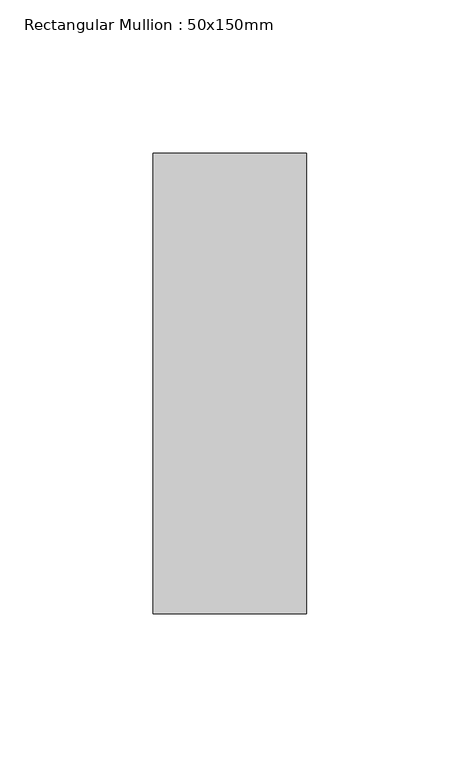
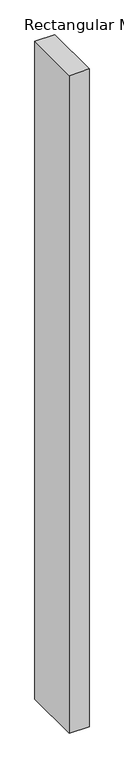
"""IFC4 building model written with IfcOpenShell, lengths in millimetres: member geometry, Rectangular Mullion : 50x150mm."""

from ifc_helpers import new_model, si_unit, frame, origin, place, context, project, spatial, polyline, outline, extrude, source, transform, mapped, element, save


def rectangular_mullion_50x150mm_86d49a4b(model_context):
    return source(origin(), model_context, "Body", "SweptSolid", [
        extrude(outline(polyline([(0.0, 75.0), (0.0, -75.0), (-50.0, -75.0), (-50.0, 75.0), (0.0, 75.0)])), frame((0.0, 0.0, -1755.0), z_axis=(0.0, 0.0, 1.0), x_axis=(1.0, 0.0, 0.0)), (0.0, 0.0, 1.0), 1755.0),
    ])


if __name__ == "__main__":
    model = new_model("IFC4")
    model_context = context("Model", 3, world=origin())
    ifc_project = project(units=[si_unit("LENGTHUNIT", "METRE", prefix="MILLI")], contexts=[model_context])
    site = spatial("IfcSite", under=ifc_project)
    building = spatial("IfcBuilding", under=site)
    placement = place(None, origin())
    rectangular_mullion_50x150mm_shape = rectangular_mullion_50x150mm_86d49a4b(model_context)
    element("IfcMember", 1, ObjectType="Rectangular Mullion : 50x150mm", at=placement, inside=building, context=model_context, shape_type="MappedRepresentation", body=[
        mapped(rectangular_mullion_50x150mm_shape, transform((0.0, 0.0, 0.0), x_axis=(1.0, 0.0, 0.0), y_axis=(0.0, 1.0, 0.0), z_axis=(0.0, 0.0, 1.0))),
    ])
    save(model, "model.ifc")

# Revit data of these elements
# Type "Rectangular Mullion : 50x150mm"
#   Keynote = "H11"
#   built-in parameter 1007304 = 0.492126 (stored number, unit not read)
#   built-in parameter 1007301 = 0.082021 (stored number, unit not read)
#   built-in parameter 1007300 = 0.082021 (stored number, unit not read)
# Element 1 (IfcMember, "Rectangular Mullion : 50x150mm")
#   Materials on its faces: "Aluminium"
# Materials
#   "Aluminium": class "Metal", colour RGB 247 247 247, transparency 0, Description = "Aluminium 6061", Cost = 0
